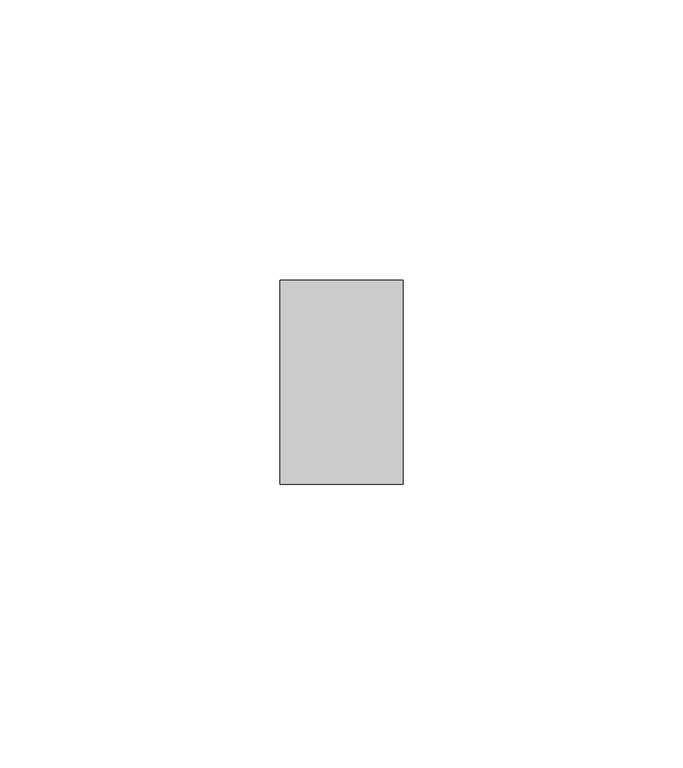
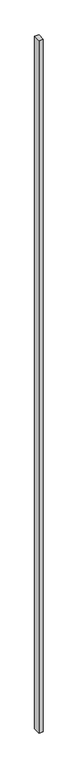
"""IFC4 building model written with IfcOpenShell, lengths in millimetres: proxy geometry, Generic Models 11:Generic Models 1:306267:Generic Models 1:306267 : Generic Models 11:Generic Models 1:306267:300405:Generic Models 1:306267:Generic Models 1:306267 : Generic Models 11:Generic Models 1:306267:300405 : Generic Models 11:Generic Models 1:306267:Generic Models 1:306267 : Generic Models 11:Generic Models 1:306267:300405:2 : Generic Models 11:Generic Models 1:306267:Generic Models 1:306267 : Generic Models 11:Generic Models 1:306267:300405:Generic Models 1:306267:Generic Models 1:306267 : Generic Models 11:Generic Models 1:306267:300405 : Generic Models 11:Generic Models 1:306267:Generic Models 1:306267 : Generic Models 11:Generic Models 1:306267:300405:300182."""

from ifc_helpers import new_model, si_unit, origin, origin_with_axes, place, context, project, spatial, polyline, outline, extrude, source, transform, mapped, element, save


def generic_models_b2f98fdd(model_context):
    return source(origin(), model_context, "Body", "SweptSolid", [
        extrude(outline(polyline([(592777.8856601, -579042.7770224), (592777.8856601, -579079.2557458), (592755.8818597, -579079.2557458), (592755.8818597, -579042.7770224), (592777.8856601, -579042.7770224)])), origin_with_axes(), (0.0, 0.0, 1.0), 3689.35),
    ])


if __name__ == "__main__":
    model = new_model("IFC4")
    model_context = context("Model", 3, world=origin())
    ifc_project = project(units=[si_unit("LENGTHUNIT", "METRE", prefix="MILLI")], contexts=[model_context])
    site = spatial("IfcSite", under=ifc_project)
    building = spatial("IfcBuilding", under=site)
    placement = place(None, origin())
    generic_models_shape = generic_models_b2f98fdd(model_context)
    element("IfcBuildingElementProxy", 1, Name="Generic Models 11:Generic Models 1:306267:Generic Models 1:306267 : Generic Models 11:Generic Models 1:306267:300405:Generic Models 1:306267:Generic Models 1:306267 : Generic Models 11:Generic Models 1:306267:300405 : Generic Models 11:Generic Models 1:306267:Generic Models 1:306267 : Generic Models 11:Generic Models 1:306267:300405:2 : Generic Models 11:Generic Models 1:306267:Generic Models 1:306267 : Generic Models 11:Generic Models 1:306267:300405:Generic Models 1:306267:Generic Models 1:306267 : Generic Models 11:Generic Models 1:306267:300405 : Generic Models 11:Generic Models 1:306267:Generic Models 1:306267 : Generic Models 11:Generic Models 1:306267:300405:300182", ObjectType="Generic Models 11:Generic Models 1:306267:Generic Models 1:306267 : Generic Models 11:Generic Models 1:306267:300405:Generic Models 1:306267:Generic Models 1:306267 : Generic Models 11:Generic Models 1:306267:300405 : Generic Models 11:Generic Models 1:306267:Generic Models 1:306267 : Generic Models 11:Generic Models 1:306267:300405:2 : Generic Models 11:Generic Models 1:306267:Generic Models 1:306267 : Generic Models 11:Generic Models 1:306267:300405:Generic Models 1:306267:Generic Models 1:306267 : Generic Models 11:Generic Models 1:306267:300405 : Generic Models 11:Generic Models 1:306267:Generic Models 1:306267 : Generic Models 11:Generic Models 1:306267:300405:300182", at=placement, inside=building, context=model_context, shape_type="MappedRepresentation", body=[
        mapped(generic_models_shape, transform((0.0, 0.0, 0.0), x_axis=(1.0, 0.0, 0.0), y_axis=(0.0, 1.0, 0.0), z_axis=(0.0, 0.0, 1.0))),
    ])
    save(model, "model.ifc")

# Revit data of these elements
# Type "Generic Models 11:Generic Models 1:306267:Generic Models 1:306267 : Generic Models 11:Generic Models 1:306267:300405:Generic Models 1:306267:Generic Models 1:306267 : Generic Models 11:Generic Models 1:306267:300405 : Generic Models 11:Generic Models 1:306267:Generic Models 1:306267 : Generic Models 11:Generic Models 1:306267:300405:2 : Generic Models 11:Generic Models 1:306267:Generic Models 1:306267 : Generic Models 11:Generic Models 1:306267:300405:Generic Models 1:306267:Generic Models 1:306267 : Generic Models 11:Generic Models 1:306267:300405 : Generic Models 11:Generic Models 1:306267:Generic Models 1:306267 : Generic Models 11:Generic Models 1:306267:300405:300182"
#   NameOverride = "Generic Models 11:Generic Models 1:306267:Generic Models 1:306267 : Generic Models 11:Generic Models 1:306267:300405:Generic Models 1:306267:Generic Models 1:306267 : Generic Models 11:Generic Models 1:306267:300405 : Generic Models 11:Generic Models 1:306267:Generic Models 1:306267 : Generic Models 11:Generic Models 1:306267:300405:300182"
#   ObjectTypeOverride = "Generic Models 1:306267:Generic Models 1:306267 : Generic Models 11:Generic Models 1:306267:300405 : Generic Models 11:Generic Models 1:306267:Generic Models 1:306267 : Generic Models 11:Generic Models 1:306267:300405"
#   Reference = "Generic Models 1"
#   Tag = "300182"
# Element 1 (IfcBuildingElementProxy, "Generic Models 11:Generic Models 1:306267:Generic Models 1:306267 : Generic Models 11:Generic Models 1:306267:300405:Generic Models 1:306267:Generic Models 1:306267 : Generic Models 11:Generic Models 1:306267:300405 : Generic Models 11:Generic Models 1:306267:Generic Models 1:306267 : Generic Models 11:Generic Models 1:306267:300405:2 : Generic Models 11:Generic Models 1:306267:Generic Models 1:306267 : Generic Models 11:Generic Models 1:306267:300405:Generic Models 1:306267:Generic Models 1:306267 : Generic Models 11:Generic Models 1:306267:300405 : Generic Models 11:Generic Models 1:306267:Generic Models 1:306267 : Generic Models 11:Generic Models 1:306267:300405:300182")
#   Materials on its faces: "PRESSURE TREATED WOOD BLOCKING - SIZE AS NECESSARY"
# Materials
#   "PRESSURE TREATED WOOD BLOCKING - SIZE AS NECESSARY": class "Wood", colour RGB 144 113 62, transparency 0, Description = "Pinus Echinata", Cost = 0
